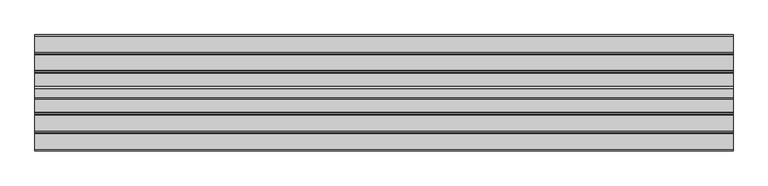
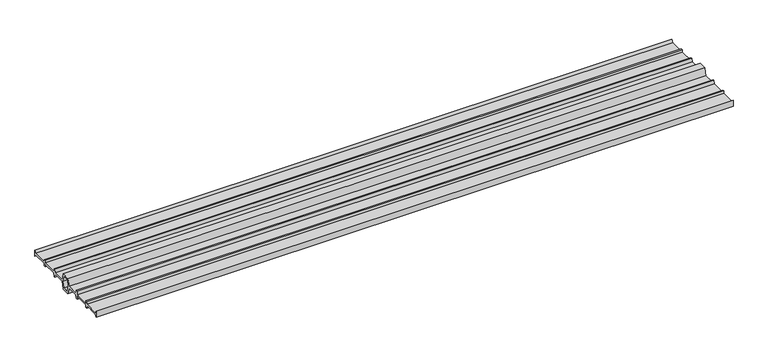
"""IFC4 building model written with IfcOpenShell, lengths in millimetres: proxy geometry, TN_Гидрошпонка ТН Фундамент : Гидрошпонка ТН Фундамент ДШ-В-250."""

from ifc_helpers import new_model, si_unit, frame, origin, place, context, project, spatial, polyline, outline, extrude, source, transform, mapped, element, save


def specialty_equipment_4845879d(model_context):
    return source(origin(), model_context, "Body", "SweptSolid", [
        extrude(outline(polyline([(-83.280218, -5.7544352), (-86.719782, -5.7544352), (-87.7344441, 0.0), (-121.5809483, 0.0), (-125.0, -5.5044352), (-125.0, 9.4955648), (-121.5809483, 3.9911296), (-87.7344441, 3.9911296), (-86.719782, 9.7455648), (-83.280218, 9.7455648), (-82.2655559, 3.9911296), (-48.0288318, 3.9911296), (-46.7513068, 11.75), (-43.2486932, 11.75), (-41.9722041, 3.9974211), (-14.1057388, 3.9974211), (-9.5980762, 20.8202469), (9.5980762, 20.8202469), (14.1057388, 3.9974211), (41.9722041, 3.9974211), (43.2486932, 11.75), (46.7513068, 11.75), (48.0288318, 3.9911296), (82.2644465, 3.9911296), (83.280218, 9.7518563), (86.719782, 9.7518563), (87.7355535, 3.9911296), (121.5809483, 3.9911296), (125.0, 9.4955648), (125.0, -5.5044352), (121.5809483, 0.0), (87.7344441, 0.0), (86.719782, -5.7544352), (83.280218, -5.7544352), (82.2655559, 0.0), (48.1139579, 0.0), (46.7513068, -8.2758715), (43.2486932, -8.2758715), (41.8860421, 0.0), (14.1057388, 0.0), (9.5980762, -16.8228258), (-9.5980762, -16.8228258), (-14.1057388, 0.0), (-41.8860421, 0.0), (-43.2486932, -8.2758715), (-46.7513068, -8.2758715), (-48.1139579, 0.0), (-82.2655559, 0.0), (-83.280218, -5.7544352)]), holes=[polyline([(-9.5720905, 2.3987105), (-5.7614413, -11.8228258), (5.7614413, -11.8228258), (9.5720905, 2.3987105), (5.9758006, 15.8202469), (-5.9758006, 15.8202469), (-9.5720905, 2.3987105)])]), frame((0.0, 0.0, 0.0), z_axis=(1.0, 0.0, 0.0), x_axis=(0.0, 1.0, 0.0)), (0.0, 0.0, 1.0), 1500.0),
    ])


if __name__ == "__main__":
    model = new_model("IFC4")
    model_context = context("Model", 3, world=origin())
    ifc_project = project(units=[si_unit("LENGTHUNIT", "METRE", prefix="MILLI")], contexts=[model_context])
    site = spatial("IfcSite", under=ifc_project)
    building = spatial("IfcBuilding", under=site)
    placement = place(None, origin())
    specialty_equipment_shape = specialty_equipment_4845879d(model_context)
    element("IfcBuildingElementProxy", 1, Name="TN_Гидрошпонка ТН Фундамент : Гидрошпонка ТН Фундамент ДШ-В-250", ObjectType="TN_Гидрошпонка ТН Фундамент : Гидрошпонка ТН Фундамент ДШ-В-250", at=placement, inside=building, context=model_context, shape_type="MappedRepresentation", body=[
        mapped(specialty_equipment_shape, transform((0.0, 0.0, 0.0), x_axis=(1.0, 0.0, 0.0), y_axis=(0.0, 1.0, 0.0), z_axis=(0.0, 0.0, 1.0))),
    ])
    save(model, "model.ifc")

# Revit data of these elements
# Type "TN_Гидрошпонка ТН Фундамент : Гидрошпонка ТН Фундамент ДШ-В-250"
#   Description = "Внутренние гидроизоляционные шпонки ТН Фундамент ДШ-В предназначены для герметизации деформационных швов бетонирования при строительстве подземных и заглубленных конструкций зданий и сооружений различного назначения и класса ответственности."
#   Type Comments = "п.м."
#   Manufacturer = "ТехноНИКОЛЬ"
#   URL = "https://nav.tn.ru/catalog/gidroizolyatsiya/komplektatsiya-dlya-gidroizolyatsii/gidroshponki-tekhnonikol-fundament-dsh-v/"
#   ADSK_Примечание = ""
#   ADSK_Обозначение [instance default] = "ТехноНИКОЛЬ"
#   ADSK_Наименование = "Гидрошпонка ТН Фундамент ДШ-В-250"
#   ADSK_Масса_Текст = ""
#   ADSK_Марка = ""
#   ADSK_Код изделия = "66669"
#   ADSK_Завод-изготовитель [instance default] = "ТехноНИКОЛЬ"
#   ADSK_Единица измерения [instance default] = "п.м."
#   ADSK_Группирование = "Гидрошпонки"
#   ADSK_URL страницы изделия = "https://nav.tn.ru/catalog/gidroizolyatsiya/komplektatsiya-dlya-gidroizolyatsii/gidroshponki-tekhnonikol-fundament-dsh-v/"
#   ADSK_URL документации изделия = "https://nav.tn.ru/upload/iblock/28f/fdn3hm8k6c3nnk1qf6d2lbujw61o7ba5/Tekhlist-7.398_Gidroshponki-TN-Fundament-DSH_V_RU_ru.pdf"
#   built-in parameter 1001306 [instance default] = 3.28084 (stored number, unit not read)
#   ADSK_Размер_Длина [instance default] = 1000 mm
#   ADSK_Количество [instance default] = 1
#   Гидрошпонка ТН Фундамент ТШ-Н-210 = no
#   Гидрошпонка ТН Фундамент ДШП-В-50 = no
#   Гидрошпонка ТН Фундамент ДШП-В-20 = no
#   Гидрошпонка ТН Фундамент ДШ-В-280 = no
#   Гидрошпонка ТН Фундамент ДШ-В-250 = yes
#   Гидрошпонка ТН Фундамент ТШ-В-250 = no
#   Гидрошпонка ТН Фундамент ТПС-В 140-1 = no
#   Гидрошпонка ТН Фундамент ДШ-Н-280 = no
#   Гидрошпонка ТН Фундамент ДШ-Н-250 = no
#   Гидрошпонка ТН Фундамент ТПС-В 100-2 = no
#   Гидрошпонка ТН Фундамент ТШ-Н-250 = no
#   Гидрошпонка ТН Фундамент ТШ-В-210 = no
#   Материал = TN_ПВХ_Черный
#   Default Elevation = 0
# Element 1 (IfcBuildingElementProxy, "TN_Гидрошпонка ТН Фундамент : Гидрошпонка ТН Фундамент ДШ-В-250")
#   built-in parameter 1001306 = 4.92126 (stored number, unit not read)
#   ADSK_Размер_Длина = 1500 mm
#   ADSK_Количество = 1.5
#   Materials on its faces: "TN_ПВХ_Черный"
# Materials
#   "TN_ПВХ_Черный": class "Типовые", colour RGB 48 48 48, transparency 0, Cost = 0
